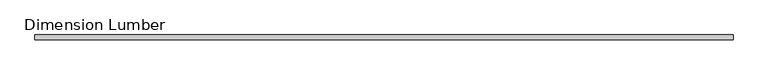
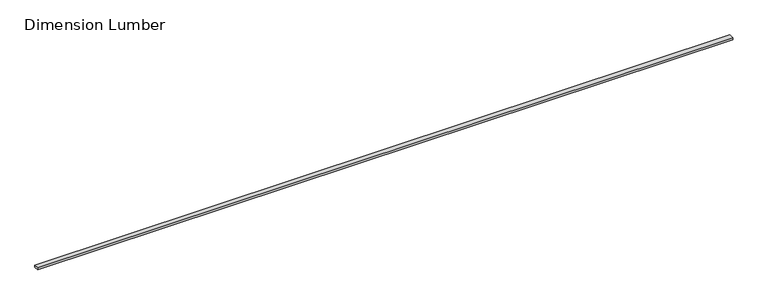
"""IFC4 building model written with IfcOpenShell, lengths in millimetres: beam geometry, Dimension Lumber : Top Supporting Lumbers."""

import ifcopenshell
import ifcopenshell.guid

model = None  # the IFC model being written
_history = None  # IfcOwnerHistory: only IFC2X3 demands one
_inside = {}  # id of a spatial element -> (the spatial element, [elements in it])
_under = {}  # id of a project, library or spatial element -> (it, [spatial elements below it])
_declared = {}  # id of a project -> (the project, [libraries it declares])
_typed = {}  # id of a type object -> (the type object, [elements of that type])
_made_of = {}  # id of a material, layer set ... -> (it, [elements and type objects made of it])


def new_model(schema):
    """Start an empty IFC model of exactly this schema.

    Asked for "IFC4X3", IfcOpenShell would pick the latest addendum, in which some entities
    have other attributes; the version numbers below select the first issue.
    IFC2X3 requires an IfcOwnerHistory on every rooted entity: one is made here for all.
    """
    global model, _history
    if schema == "IFC4X3":
        model = ifcopenshell.file(schema_version=(4, 3, 0, 0))
    else:
        model = ifcopenshell.file(schema=schema)
    _inside.clear()
    _under.clear()
    _declared.clear()
    _typed.clear()
    _made_of.clear()
    _history = None
    if model.schema == "IFC2X3":
        org = make("IfcOrganization", Name="unknown")
        user = make(
            "IfcPersonAndOrganization",
            ThePerson=make("IfcPerson", FamilyName="unknown"),
            TheOrganization=org,
        )
        app = make(
            "IfcApplication",
            ApplicationDeveloper=org,
            Version="unknown",
            ApplicationFullName="unknown",
            ApplicationIdentifier="unknown",
        )
        _history = make(
            "IfcOwnerHistory",
            OwningUser=user,
            OwningApplication=app,
            ChangeAction="ADDED",
            CreationDate=0,
        )
    return model


def make(cls, **values):
    """One entity of the class cls with the attributes given. An attribute that is None is left unset."""
    return model.create_entity(
        cls, **{name: value for name, value in values.items() if value is not None}
    )


def rooted(cls, **values):
    """An entity with a GlobalId (a new one), such as an element, a storey or a relation."""
    return make(cls, GlobalId=ifcopenshell.guid.new(), OwnerHistory=_history, **values)


def si_unit(unit_type, name, prefix=None):
    """IfcSIUnit, for example si_unit("LENGTHUNIT", "METRE", prefix="MILLI")."""
    return make("IfcSIUnit", UnitType=unit_type, Prefix=prefix, Name=name)


def assignment(units):
    """IfcUnitAssignment: the units of a project."""
    return None if units is None else make("IfcUnitAssignment", Units=units)


def point(xyz):
    """IfcCartesianPoint."""
    return None if xyz is None else make("IfcCartesianPoint", Coordinates=xyz)


def direction(xyz):
    """IfcDirection."""
    return None if xyz is None else make("IfcDirection", DirectionRatios=xyz)


def frame(location, z_axis=None, x_axis=None):
    """IfcAxis2Placement3D, a coordinate frame: its origin and axes. An axis left out is left unset."""
    return make(
        "IfcAxis2Placement3D",
        Location=point(location),
        Axis=direction(z_axis),
        RefDirection=direction(x_axis),
    )


def origin():
    """The frame at (0, 0, 0) with its axes left unset."""
    return frame((0.0, 0.0, 0.0))


def place(relative_to, where):
    """IfcLocalPlacement: puts the frame where relative to a parent placement (None: the world)."""
    return make(
        "IfcLocalPlacement", PlacementRelTo=relative_to, RelativePlacement=where
    )


def context(
    kind, dimensions, precision=None, world=None, true_north=None, identifier=None
):
    """IfcGeometricRepresentationContext, for example the 3D "Model" context."""
    return make(
        "IfcGeometricRepresentationContext",
        ContextIdentifier=identifier,
        ContextType=kind,
        CoordinateSpaceDimension=dimensions,
        Precision=precision,
        WorldCoordinateSystem=world,
        TrueNorth=true_north,
    )


def project(units=None, contexts=None):
    """IfcProject with its units and contexts."""
    return rooted(
        "IfcProject",
        Name="project",
        RepresentationContexts=contexts,
        UnitsInContext=assignment(units),
    )


def spatial(cls, under=None, at=None, **own):
    """A site, building, storey or space (cls), placed at a placement, below another one or the project."""
    s = rooted(cls, ObjectPlacement=at, **own)
    if under is not None:
        _under.setdefault(under.id(), (under, []))[1].append(s)
    return s


def polyline(points):
    """IfcPolyline through the points."""
    return make("IfcPolyline", Points=[point(p) for p in points])


def outline(outer, holes=None, kind="AREA"):
    """IfcArbitraryClosedProfileDef: a profile drawn as a closed curve; with holes, ...WithVoids."""
    if holes is None:
        return make("IfcArbitraryClosedProfileDef", ProfileType=kind, OuterCurve=outer)
    return make(
        "IfcArbitraryProfileDefWithVoids",
        ProfileType=kind,
        OuterCurve=outer,
        InnerCurves=holes,
    )


def extrude(swept, where, along, depth):
    """IfcExtrudedAreaSolid: the profile swept, set in the frame where, extruded along a direction by depth."""
    return make(
        "IfcExtrudedAreaSolid",
        SweptArea=swept,
        Position=where,
        ExtrudedDirection=direction(along),
        Depth=depth,
    )


def shape(context_of_items, identifier, shape_type, items):
    """IfcShapeRepresentation: the items that make up one representation, for example the "Body"."""
    return make(
        "IfcShapeRepresentation",
        ContextOfItems=context_of_items,
        RepresentationIdentifier=identifier,
        RepresentationType=shape_type,
        Items=items,
    )


def source(mapping_origin, context_of_items, identifier, shape_type, items):
    """IfcRepresentationMap: a shape defined once, which mapped items show again and again."""
    return make(
        "IfcRepresentationMap",
        MappingOrigin=mapping_origin,
        MappedRepresentation=shape(context_of_items, identifier, shape_type, items),
    )


def transform(
    local_origin,
    x_axis=None,
    y_axis=None,
    z_axis=None,
    scale=None,
    scale2=None,
    scale3=None,
    uniform=True,
):
    """IfcCartesianTransformationOperator3D, or its non-uniform kind. x_axis, y_axis, z_axis: its Axis1, 2, 3."""
    if uniform:
        return make(
            "IfcCartesianTransformationOperator3D",
            Axis1=direction(x_axis),
            Axis2=direction(y_axis),
            LocalOrigin=point(local_origin),
            Scale=scale,
            Axis3=direction(z_axis),
        )
    return make(
        "IfcCartesianTransformationOperator3DnonUniform",
        Axis1=direction(x_axis),
        Axis2=direction(y_axis),
        LocalOrigin=point(local_origin),
        Scale=scale,
        Axis3=direction(z_axis),
        Scale2=scale2,
        Scale3=scale3,
    )


def mapped(mapping_source, mapping_target):
    """IfcMappedItem: shows the shape of a source again, moved by a transform."""
    return make(
        "IfcMappedItem", MappingSource=mapping_source, MappingTarget=mapping_target
    )


def made_of(thing, what):
    """Note that an element or type object is made of a material, layer set ...; save() writes the relation."""
    if what is not None:
        _made_of.setdefault(what.id(), (what, []))[1].append(thing)
    return thing


def element(
    cls,
    number,
    at=None,
    inside=None,
    cuts=None,
    type_object=None,
    material=None,
    context=None,
    identifier="Body",
    shape_type=None,
    held_by="IfcProductDefinitionShape",
    body=None,
    shapes=None,
    **own,
):
    """One element of the class cls, such as IfcWall. Its Tag is "e" and its number.

    at: its placement. inside: the storey or other place that contains it. cuts: it is an
    opening in that element (IfcRelVoidsElement). A single representation is given by context,
    identifier, shape_type and body (its items); several are given by shapes. held_by: the class
    of the entity that holds the representations. save() writes the other relations.
    """
    e = rooted(cls, Tag="e%d" % number, ObjectPlacement=at, **own)
    if body is not None:
        shapes = [shape(context, identifier, shape_type, body)]
    if shapes is not None:
        e.Representation = make(held_by, Representations=shapes)
    if inside is not None:
        _inside.setdefault(inside.id(), (inside, []))[1].append(e)
    if cuts is not None:
        rooted(
            "IfcRelVoidsElement", RelatingBuildingElement=cuts, RelatedOpeningElement=e
        )
    if type_object is not None:
        _typed.setdefault(type_object.id(), (type_object, []))[1].append(e)
    return made_of(e, material)


def aggregate(whole, parts):
    """IfcRelAggregates: a whole, such as a stair, and the parts it consists of."""
    return rooted("IfcRelAggregates", RelatingObject=whole, RelatedObjects=parts)


def save(model, path):
    """Write the relations noted so far, then the file.

    IfcRelAggregates (storeys below a building ...), IfcRelContainedInSpatialStructure (elements
    in a storey), IfcRelDefinesByType, IfcRelAssociatesMaterial and IfcRelDeclares: one each for
    every whole, place, type object, material and project.
    """
    for whole, parts in _under.values():
        aggregate(whole, parts)
    for where, things in _inside.values():
        rooted(
            "IfcRelContainedInSpatialStructure",
            RelatedElements=things,
            RelatingStructure=where,
        )
    for kind, things in _typed.values():
        rooted("IfcRelDefinesByType", RelatedObjects=things, RelatingType=kind)
    for what, things in _made_of.values():
        rooted("IfcRelAssociatesMaterial", RelatedObjects=things, RelatingMaterial=what)
    for by, libraries in _declared.values():
        rooted("IfcRelDeclares", RelatingContext=by, RelatedDefinitions=libraries)
    model.write(path)


def dimension_lumber_2a703131(model_context):
    return source(origin(), model_context, "Body", "SweptSolid", [
        extrude(outline(polyline([(6275.3875, 44.45), (6275.3875, -44.45), (-6338.8875, -44.45), (-6338.8875, 44.45), (6275.3875, 44.45)])), frame((0.0, 0.0, -19.05), z_axis=(0.0, 0.0, 1.0), x_axis=(1.0, 0.0, 0.0)), (0.0, 0.0, 1.0), 38.1),
    ])


if __name__ == "__main__":
    model = new_model("IFC4")
    model_context = context("Model", 3, world=origin())
    ifc_project = project(units=[si_unit("LENGTHUNIT", "METRE", prefix="MILLI")], contexts=[model_context])
    site = spatial("IfcSite", under=ifc_project)
    building = spatial("IfcBuilding", under=site)
    placement = place(None, origin())
    dimension_lumber_shape = dimension_lumber_2a703131(model_context)
    element("IfcBeam", 1, ObjectType="Dimension Lumber : Top Supporting Lumbers", at=placement, inside=building, context=model_context, shape_type="MappedRepresentation", body=[
        mapped(dimension_lumber_shape, transform((0.0, 0.0, 0.0), x_axis=(1.0, 0.0, 0.0), y_axis=(0.0, 1.0, 0.0), z_axis=(0.0, 0.0, 1.0))),
    ])
    save(model, "model.ifc")

# Revit data of these elements
# Type "Dimension Lumber : Top Supporting Lumbers"
#   Assembly Code = "B10"
#   A = 0.0364583 SF
#   Length [instance default] = 5' - 0"
#   b = 0' - 3 1/2"
#   d = 0' - 1 1/2"
#   Structural Material [instance default] = Softwood, Lumber
# Element 1 (IfcBeam, "Dimension Lumber : Top Supporting Lumbers")
#   Structural Material = Douglas Fir #2
#   Materials on its faces: "Douglas Fir #2"
# Materials
#   "Softwood, Lumber": class "Wood", colour RGB 223 192 134, transparency 0, Description = "Pinus Echinata", Cost = 0
#   "Douglas Fir #2": class "Wood", colour RGB 223 192 134, transparency 0, Description = "Pinus Echinata", Cost = 0
